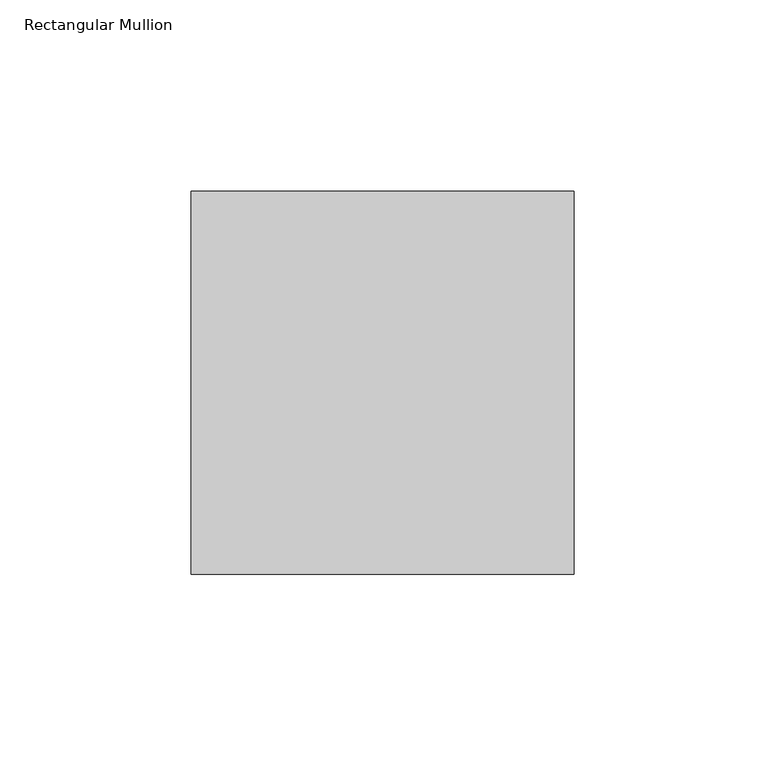
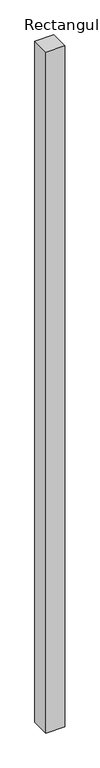
"""IFC4 building model written with IfcOpenShell, lengths in millimetres: member geometry, Rectangular Mullion : 알루미늄_Rectangular Cap_100 x100."""

from ifc_helpers import new_model, si_unit, frame, origin, place, context, project, spatial, polyline, outline, extrude, source, transform, mapped, element, save


def rectangular_mullion_9ba7f3a8(model_context):
    return source(origin(), model_context, "Body", "SweptSolid", [
        extrude(outline(polyline([(0.0, 50.0), (0.0, -50.0), (-100.0, -50.0), (-100.0, 50.0), (0.0, 50.0)])), frame((0.0, 0.0, -3775.0), z_axis=(0.0, 0.0, 1.0), x_axis=(1.0, 0.0, 0.0)), (0.0, 0.0, 1.0), 3775.0),
    ])


if __name__ == "__main__":
    model = new_model("IFC4")
    model_context = context("Model", 3, world=origin())
    ifc_project = project(units=[si_unit("LENGTHUNIT", "METRE", prefix="MILLI")], contexts=[model_context])
    site = spatial("IfcSite", under=ifc_project)
    building = spatial("IfcBuilding", under=site)
    placement = place(None, origin())
    rectangular_mullion_shape = rectangular_mullion_9ba7f3a8(model_context)
    element("IfcMember", 1, ObjectType="Rectangular Mullion : 알루미늄_Rectangular Cap_100 x100", at=placement, inside=building, context=model_context, shape_type="MappedRepresentation", body=[
        mapped(rectangular_mullion_shape, transform((0.0, 0.0, 0.0), x_axis=(1.0, 0.0, 0.0), y_axis=(0.0, 1.0, 0.0), z_axis=(0.0, 0.0, 1.0))),
    ])
    save(model, "model.ifc")

# Revit data of these elements
# Type "Rectangular Mullion : 알루미늄_Rectangular Cap_100 x100"
#   built-in parameter 1007304 = 0.328084 (stored number, unit not read)
#   built-in parameter 1007301 = 0.164042 (stored number, unit not read)
#   built-in parameter 1007300 = 0.164042 (stored number, unit not read)
# Element 1 (IfcMember, "Rectangular Mullion : 알루미늄_Rectangular Cap_100 x100")
#   Materials on its faces: "00_Metal_Stainless Steel"
# Materials
#   "00_Metal_Stainless Steel": class "Metal", colour RGB 148 148 148, transparency 0, Description = "Steel", Cost = 0
